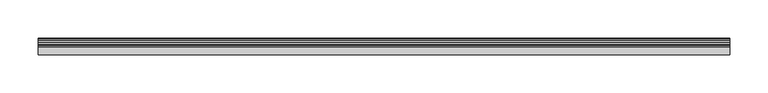
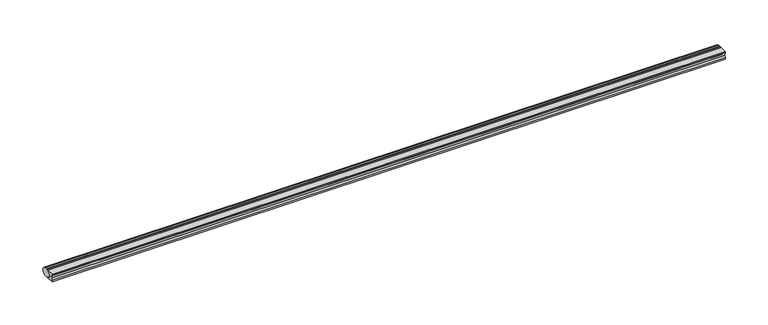
"""IFC4 building model written with IfcOpenShell, lengths in millimetres: proxy geometry, Generic Models 7:Generic Models 1:1:Generic Models 1:1 : Generic Models 7:Generic Models 1:337419:42 : Generic Models 7:Generic Models 1:1:Generic Models 1:1 : Generic Models 7:Generic Models 1:337419:306201."""

from ifc_helpers import new_model, si_unit, frame, origin, place, context, project, spatial, polyline, outline, extrude, source, transform, mapped, element, save


def generic_models_9bd0b28a(model_context):
    return source(origin(), model_context, "Body", "SweptSolid", [
        extrude(outline(polyline([(-579108.3321247, 3712.6918825), (-579109.7738584, 3712.0444579), (-579111.9685584, 3710.2286587), (-579112.9746831, 3707.9657961), (-579112.6348335, 3705.6098738), (-579111.002176, 3703.5294543), (-579108.3321247, 3702.05), (-579118.1663841, 3702.05), (-579117.5338899, 3703.66851), (-579117.0081875, 3707.3709413), (-579117.5338899, 3711.0733725), (-579118.1663841, 3712.6918825), (-579108.3321247, 3712.6918825)])), frame((592795.5032101, 0.0, 0.0), z_axis=(1.0, 0.0, 0.0), x_axis=(0.0, 1.0, 0.0)), (0.0, 0.0, 1.0), 910.0612812),
        extrude(outline(polyline([(-579102.5949207, 3712.5584754), (-579099.394623, 3711.5310207), (-579097.1799483, 3709.6796112), (-579096.3895401, 3707.3709413), (-579097.1799483, 3705.0622714), (-579099.394623, 3703.2108619), (-579102.5949207, 3702.1834071), (-579104.370952, 3702.05), (-579106.1469832, 3702.1834071), (-579109.3472809, 3703.2108619), (-579111.5619556, 3705.0622714), (-579112.3523639, 3707.3709413), (-579111.5619556, 3709.6796112), (-579109.3472809, 3711.5310207), (-579106.1469832, 3712.5584754), (-579104.370952, 3712.6918825), (-579102.5949207, 3712.5584754)])), frame((592795.5032101, 0.0, 0.0), z_axis=(1.0, 0.0, 0.0), x_axis=(0.0, 1.0, 0.0)), (0.0, 0.0, 1.0), 910.0612812),
    ])


if __name__ == "__main__":
    model = new_model("IFC4")
    model_context = context("Model", 3, world=origin())
    ifc_project = project(units=[si_unit("LENGTHUNIT", "METRE", prefix="MILLI")], contexts=[model_context])
    site = spatial("IfcSite", under=ifc_project)
    building = spatial("IfcBuilding", under=site)
    placement = place(None, origin())
    generic_models_shape = generic_models_9bd0b28a(model_context)
    element("IfcBuildingElementProxy", 1, Name="Generic Models 7:Generic Models 1:1:Generic Models 1:1 : Generic Models 7:Generic Models 1:337419:42 : Generic Models 7:Generic Models 1:1:Generic Models 1:1 : Generic Models 7:Generic Models 1:337419:306201", ObjectType="Generic Models 7:Generic Models 1:1:Generic Models 1:1 : Generic Models 7:Generic Models 1:337419:42 : Generic Models 7:Generic Models 1:1:Generic Models 1:1 : Generic Models 7:Generic Models 1:337419:306201", at=placement, inside=building, context=model_context, shape_type="MappedRepresentation", body=[
        mapped(generic_models_shape, transform((0.0, 0.0, 0.0), x_axis=(1.0, 0.0, 0.0), y_axis=(0.0, 1.0, 0.0), z_axis=(0.0, 0.0, 1.0))),
    ])
    save(model, "model.ifc")

# Revit data of these elements
# Type "Generic Models 7:Generic Models 1:1:Generic Models 1:1 : Generic Models 7:Generic Models 1:337419:42 : Generic Models 7:Generic Models 1:1:Generic Models 1:1 : Generic Models 7:Generic Models 1:337419:306201"
#   NameOverride = "Generic Models 7:Generic Models 1:1:Generic Models 1:1 : Generic Models 7:Generic Models 1:337419:306201"
#   ObjectTypeOverride = "Generic Models 1:1 : Generic Models 7:Generic Models 1:337419"
#   Reference = "Generic Models 1"
#   Tag = "306201"
# Element 1 (IfcBuildingElementProxy, "Generic Models 7:Generic Models 1:1:Generic Models 1:1 : Generic Models 7:Generic Models 1:337419:42 : Generic Models 7:Generic Models 1:1:Generic Models 1:1 : Generic Models 7:Generic Models 1:337419:306201")
#   Materials on its faces: "SEMI-RIGID EPOXY SEALANT W/ BACKROD (REMOVE TEMP. JOINT FORM)"
# Materials
#   "SEMI-RIGID EPOXY SEALANT W/ BACKROD (REMOVE TEMP. JOINT FORM)": class "Unassigned", colour RGB 120 120 120, transparency 0, Cost = 0
